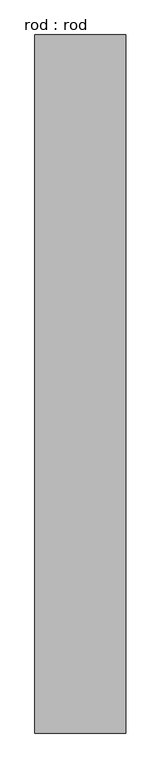
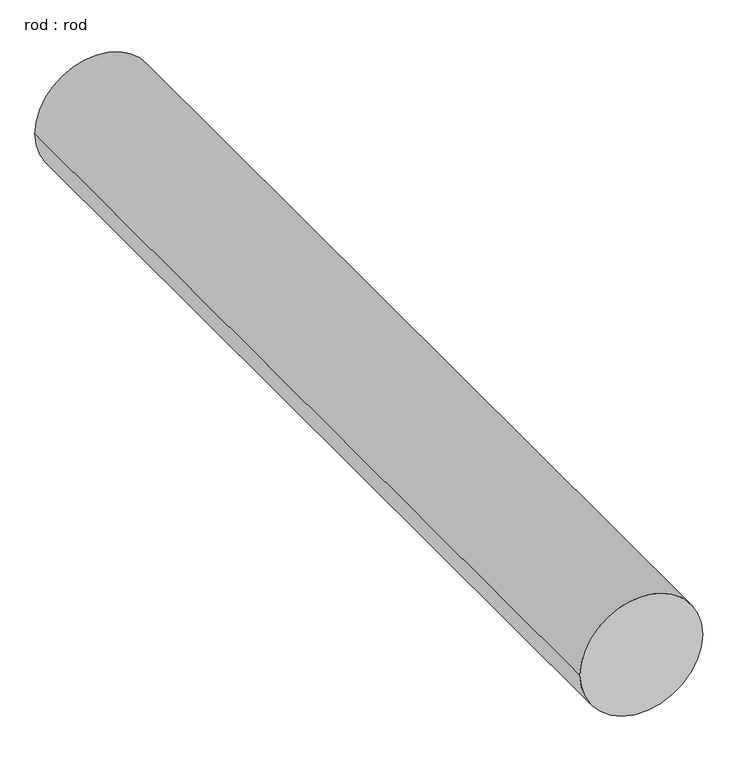
"""IFC4 building model written with IfcOpenShell, lengths in millimetres: proxy geometry, rod : rod."""

from ifc_helpers import new_model, si_unit, point, frame, frame_2d, origin, place, context, project, spatial, circle_curve, trimmed, segment, composite_curve, outline, extrude, source, transform, mapped, element, save


def rod_rod_4b894fce(model_context):
    return source(origin(), model_context, "Body", "SweptSolid", [
        extrude(outline(composite_curve([segment(trimmed(circle_curve(frame_2d((0.0108462, 0.0)), 200.0), [point((0.0108462, 200.0))], [point((0.0108462, -200.0))], False, "CARTESIAN"), True, "CONTINUOUS"), segment(trimmed(circle_curve(frame_2d((0.0108462, 0.0)), 200.0), [point((0.0108462, -200.0))], [point((0.0108462, 200.0))], False, "CARTESIAN"), True, "CONTINUOUS")], self_intersect=False)), frame((0.0, 2555.2286153, 0.0), z_axis=(0.0, 1.0, 0.0), x_axis=(0.0, 0.0, 1.0)), (0.0, 0.0, 1.0), 3075.0),
    ])


if __name__ == "__main__":
    model = new_model("IFC4")
    model_context = context("Model", 3, world=origin())
    ifc_project = project(units=[si_unit("LENGTHUNIT", "METRE", prefix="MILLI")], contexts=[model_context])
    site = spatial("IfcSite", under=ifc_project)
    building = spatial("IfcBuilding", under=site)
    placement = place(None, origin())
    rod_rod_shape = rod_rod_4b894fce(model_context)
    element("IfcBuildingElementProxy", 1, Name="rod : rod", ObjectType="rod : rod", at=placement, inside=building, context=model_context, shape_type="MappedRepresentation", body=[
        mapped(rod_rod_shape, transform((0.0, 0.0, 0.0), x_axis=(1.0, 0.0, 0.0), y_axis=(0.0, 1.0, 0.0), z_axis=(0.0, 0.0, 1.0))),
    ])
    save(model, "model.ifc")

# Revit data of these elements
# Type "rod : rod"
#   Default Elevation = 0
